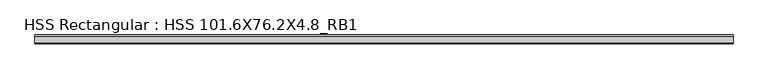
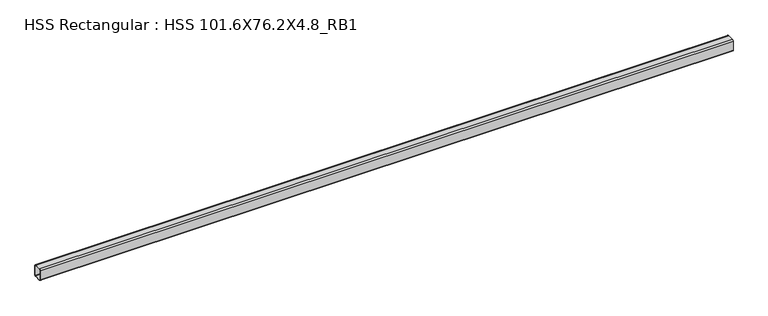
"""IFC4 building model written with IfcOpenShell, lengths in millimetres: beam geometry, HSS Rectangular : HSS 101.6X76.2X4.8_RB1."""

from ifc_helpers import new_model, si_unit, point, frame, frame_2d, origin, place, context, project, spatial, polyline, circle_curve, trimmed, segment, composite_curve, outline, extrude, source, transform, mapped, element, save


def hss_rectangular_hss_101_6x76_2x4_8_rb1_f9312058(model_context):
    return source(origin(), model_context, "Body", "SweptSolid", [
        extrude(outline(composite_curve([segment(polyline([(38.1, 41.275), (38.1, -41.275)]), True, "CONTINUOUS"), segment(trimmed(circle_curve(frame_2d((28.575, -41.275)), 9.525), [point((38.1, -41.275))], [point((28.575, -50.8))], False, "CARTESIAN"), True, "CONTINUOUS"), segment(polyline([(28.575, -50.8), (-28.575, -50.8)]), True, "CONTINUOUS"), segment(trimmed(circle_curve(frame_2d((-28.575, -41.275)), 9.525), [point((-28.575, -50.8))], [point((-38.1, -41.275))], False, "CARTESIAN"), True, "CONTINUOUS"), segment(polyline([(-38.1, -41.275), (-38.1, 41.275)]), True, "CONTINUOUS"), segment(trimmed(circle_curve(frame_2d((-28.575, 41.275)), 9.525), [point((-38.1, 41.275))], [point((-28.575, 50.8))], False, "CARTESIAN"), True, "CONTINUOUS"), segment(polyline([(-28.575, 50.8), (28.575, 50.8)]), True, "CONTINUOUS"), segment(trimmed(circle_curve(frame_2d((28.575, 41.275)), 9.525), [point((28.575, 50.8))], [point((38.1, 41.275))], False, "CARTESIAN"), True, "CONTINUOUS")], self_intersect=False), holes=[composite_curve([segment(trimmed(circle_curve(frame_2d((-28.575, 41.275)), 4.7625), [point((-28.575, 46.0375))], [point((-33.3375, 41.275))], True, "CARTESIAN"), True, "CONTINUOUS"), segment(polyline([(-33.3375, 41.275), (-33.3375, -41.275)]), True, "CONTINUOUS"), segment(trimmed(circle_curve(frame_2d((-28.575, -41.275)), 4.7625), [point((-33.3375, -41.275))], [point((-28.575, -46.0375))], True, "CARTESIAN"), True, "CONTINUOUS"), segment(polyline([(-28.575, -46.0375), (28.575, -46.0375)]), True, "CONTINUOUS"), segment(trimmed(circle_curve(frame_2d((28.575, -41.275)), 4.7625), [point((28.575, -46.0375))], [point((33.3375, -41.275))], True, "CARTESIAN"), True, "CONTINUOUS"), segment(polyline([(33.3375, -41.275), (33.3375, 41.275)]), True, "CONTINUOUS"), segment(trimmed(circle_curve(frame_2d((28.575, 41.275)), 4.7625), [point((33.3375, 41.275))], [point((28.575, 46.0375))], True, "CARTESIAN"), True, "CONTINUOUS"), segment(polyline([(28.575, 46.0375), (-28.575, 46.0375)]), True, "CONTINUOUS")], self_intersect=False)]), frame((-7484.628596, 0.0, 0.0), z_axis=(1.0, 0.0, 0.0), x_axis=(0.0, 1.0, 0.0)), (0.0, 0.0, 1.0), 5855.2008079),
    ])


if __name__ == "__main__":
    model = new_model("IFC4")
    model_context = context("Model", 3, world=origin())
    ifc_project = project(units=[si_unit("LENGTHUNIT", "METRE", prefix="MILLI")], contexts=[model_context])
    site = spatial("IfcSite", under=ifc_project)
    building = spatial("IfcBuilding", under=site)
    placement = place(None, origin())
    hss_rectangular_hss_101_6x76_2x4_8_rb1_shape = hss_rectangular_hss_101_6x76_2x4_8_rb1_f9312058(model_context)
    element("IfcBeam", 1, ObjectType="HSS Rectangular : HSS 101.6X76.2X4.8_RB1", at=placement, inside=building, context=model_context, shape_type="MappedRepresentation", body=[
        mapped(hss_rectangular_hss_101_6x76_2x4_8_rb1_shape, transform((0.0, 0.0, 0.0), x_axis=(1.0, 0.0, 0.0), y_axis=(0.0, 1.0, 0.0), z_axis=(0.0, 0.0, 1.0))),
    ])
    save(model, "model.ifc")

# Revit data of these elements
# Type "HSS Rectangular : HSS 101.6X76.2X4.8_RB1"
#   Section Name Key = "HSS 4X3X3/16"
#   Assembly Code = "B10"
#   Width = 7.62 cm
#   Wall Nominal Thickness = 0.4763 cm
#   Wall Design Thickness = 0.442 cm
#   Torsional Moment of Inertia = 260.561 cm⁴
#   Torsional Modulus = 61.2876 cm³
#   Section Area = 14.4516 cm²
#   Plastic Modulus weak axis = 40.3122 cm³
#   Plastic Modulus strong axis = 49.1612 cm³
#   Perimeter = 0.881482 m²/m
#   Outer Fillet = 0.9525 cm
#   Nominal Weight = 12.1285 kgf/m
#   Moment of Inertia weak axis = 131.529 cm⁴
#   Moment of Inertia strong axis = 205.202 cm⁴
#   Inner Fillet = 0.4763 cm
#   Height = 10.16 cm
#   Elastic Modulus weak axis = 34.4128 cm³
#   Elastic Modulus strong axis = 40.476 cm³
#   Centroid Vertical = 5.08 cm
#   Centroid Horizontal = 3.81 cm
#   Length [instance default] = 1524 mm
#   Structural Material [instance default] = Steel ASTM A500, Grade B, Rectangular and Square
#   Principal Axes Angle = 0
# Element 1 (IfcBeam, "HSS Rectangular : HSS 101.6X76.2X4.8_RB1")
#   Structural Material = Steel ASTM A992
#   Materials on its faces: "Steel ASTM A992"
# Materials
#   "Steel ASTM A500, Grade B, Rectangular and Square": class "Metal", colour RGB 199 199 199, transparency 0, Description = "Carbon steel", Cost = 0
#   "Steel ASTM A992": class "Metal", colour RGB 199 199 199, transparency 0, Description = "Structural steel 50ksi", Cost = 0
